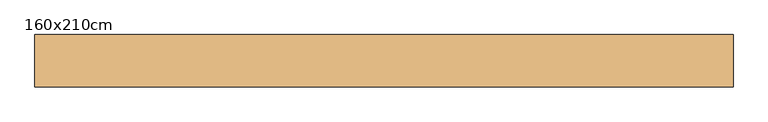
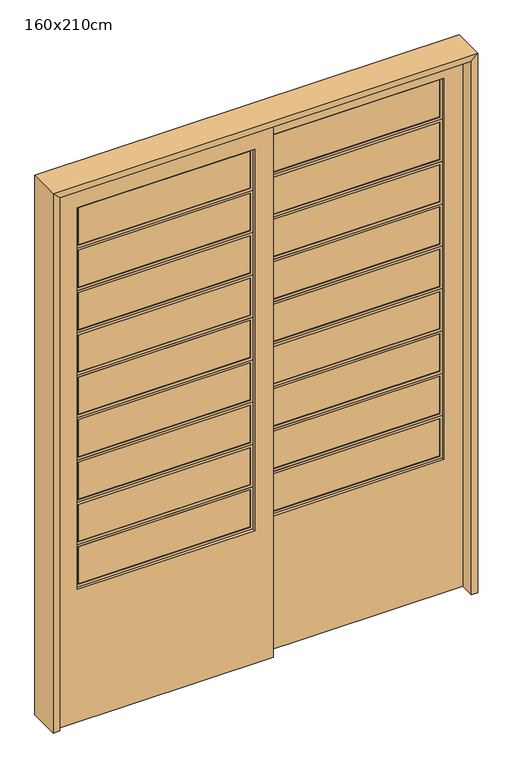
"""IFC4 building model written with IfcOpenShell, lengths in millimetres: door geometry, Porta de Correr Metálica com Divisões Horizontais : 160x210cm."""

from ifc_helpers import new_model, si_unit, frame, origin, place, context, project, spatial, polyline, outline, extrude, faceted_brep, source, transform, mapped, element, save


def door_160x210cm_b8ce621b(model_context):
    return source(origin(), model_context, "Body", "SolidModel", [
        extrude(outline(polyline([(693.0, -14.8955481), (693.0, -19.8955481), (45.0, -19.8955481), (45.0, -14.8955481), (693.0, -14.8955481)])), frame((0.0, 0.0, 1944.1111111), z_axis=(0.0, 0.0, 1.0), x_axis=(1.0, 0.0, 0.0)), (0.0, 0.0, 1.0), 149.0),
        extrude(outline(polyline([(1934.1111111, 703.0), (2103.1111111, 703.0), (2103.1111111, 35.0), (1934.1111111, 35.0), (1934.1111111, 703.0)]), holes=[polyline([(2093.1111111, 45.0), (2093.1111111, 693.0), (1944.1111111, 693.0), (1944.1111111, 45.0), (2093.1111111, 45.0)])]), frame((0.0, -22.3955481, 0.0), z_axis=(0.0, 1.0, 0.0), x_axis=(0.0, 0.0, 1.0)), (0.0, 0.0, 1.0), 10.0),
        extrude(outline(polyline([(693.0, -14.8955481), (693.0, -19.8955481), (45.0, -19.8955481), (45.0, -14.8955481), (693.0, -14.8955481)])), frame((0.0, 0.0, 1775.2222222), z_axis=(0.0, 0.0, 1.0), x_axis=(1.0, 0.0, 0.0)), (0.0, 0.0, 1.0), 149.0),
        extrude(outline(polyline([(1765.2222222, 703.0), (1934.2222222, 703.0), (1934.2222222, 35.0), (1765.2222222, 35.0), (1765.2222222, 703.0)]), holes=[polyline([(1924.2222222, 45.0), (1924.2222222, 693.0), (1775.2222222, 693.0), (1775.2222222, 45.0), (1924.2222222, 45.0)])]), frame((0.0, -22.3955481, 0.0), z_axis=(0.0, 1.0, 0.0), x_axis=(0.0, 0.0, 1.0)), (0.0, 0.0, 1.0), 10.0),
        extrude(outline(polyline([(693.0, -14.8955481), (693.0, -19.8955481), (45.0, -19.8955481), (45.0, -14.8955481), (693.0, -14.8955481)])), frame((0.0, 0.0, 1606.3333333), z_axis=(0.0, 0.0, 1.0), x_axis=(1.0, 0.0, 0.0)), (0.0, 0.0, 1.0), 149.0),
        extrude(outline(polyline([(1596.3333333, 703.0), (1765.3333333, 703.0), (1765.3333333, 35.0), (1596.3333333, 35.0), (1596.3333333, 703.0)]), holes=[polyline([(1755.3333333, 45.0), (1755.3333333, 693.0), (1606.3333333, 693.0), (1606.3333333, 45.0), (1755.3333333, 45.0)])]), frame((0.0, -22.3955481, 0.0), z_axis=(0.0, 1.0, 0.0), x_axis=(0.0, 0.0, 1.0)), (0.0, 0.0, 1.0), 10.0),
        extrude(outline(polyline([(693.0, -14.8955481), (693.0, -19.8955481), (45.0, -19.8955481), (45.0, -14.8955481), (693.0, -14.8955481)])), frame((0.0, 0.0, 1437.4444444), z_axis=(0.0, 0.0, 1.0), x_axis=(1.0, 0.0, 0.0)), (0.0, 0.0, 1.0), 149.0),
        extrude(outline(polyline([(1427.4444444, 703.0), (1596.4444444, 703.0), (1596.4444444, 35.0), (1427.4444444, 35.0), (1427.4444444, 703.0)]), holes=[polyline([(1586.4444444, 45.0), (1586.4444444, 693.0), (1437.4444444, 693.0), (1437.4444444, 45.0), (1586.4444444, 45.0)])]), frame((0.0, -22.3955481, 0.0), z_axis=(0.0, 1.0, 0.0), x_axis=(0.0, 0.0, 1.0)), (0.0, 0.0, 1.0), 10.0),
        extrude(outline(polyline([(693.0, -14.8955481), (693.0, -19.8955481), (45.0, -19.8955481), (45.0, -14.8955481), (693.0, -14.8955481)])), frame((0.0, 0.0, 1268.5555556), z_axis=(0.0, 0.0, 1.0), x_axis=(1.0, 0.0, 0.0)), (0.0, 0.0, 1.0), 149.0),
        extrude(outline(polyline([(1258.5555556, 703.0), (1427.5555556, 703.0), (1427.5555556, 35.0), (1258.5555556, 35.0), (1258.5555556, 703.0)]), holes=[polyline([(1417.5555556, 45.0), (1417.5555556, 693.0), (1268.5555556, 693.0), (1268.5555556, 45.0), (1417.5555556, 45.0)])]), frame((0.0, -22.3955481, 0.0), z_axis=(0.0, 1.0, 0.0), x_axis=(0.0, 0.0, 1.0)), (0.0, 0.0, 1.0), 10.0),
        extrude(outline(polyline([(693.0, -14.8955481), (693.0, -19.8955481), (45.0, -19.8955481), (45.0, -14.8955481), (693.0, -14.8955481)])), frame((0.0, 0.0, 1099.6666667), z_axis=(0.0, 0.0, 1.0), x_axis=(1.0, 0.0, 0.0)), (0.0, 0.0, 1.0), 149.0),
        extrude(outline(polyline([(1089.6666667, 703.0), (1258.6666667, 703.0), (1258.6666667, 35.0), (1089.6666667, 35.0), (1089.6666667, 703.0)]), holes=[polyline([(1248.6666667, 45.0), (1248.6666667, 693.0), (1099.6666667, 693.0), (1099.6666667, 45.0), (1248.6666667, 45.0)])]), frame((0.0, -22.3955481, 0.0), z_axis=(0.0, 1.0, 0.0), x_axis=(0.0, 0.0, 1.0)), (0.0, 0.0, 1.0), 10.0),
        extrude(outline(polyline([(693.0, -14.8955481), (693.0, -19.8955481), (45.0, -19.8955481), (45.0, -14.8955481), (693.0, -14.8955481)])), frame((0.0, 0.0, 930.7777778), z_axis=(0.0, 0.0, 1.0), x_axis=(1.0, 0.0, 0.0)), (0.0, 0.0, 1.0), 149.0),
        extrude(outline(polyline([(920.7777778, 703.0), (1089.7777778, 703.0), (1089.7777778, 35.0), (920.7777778, 35.0), (920.7777778, 703.0)]), holes=[polyline([(1079.7777778, 45.0), (1079.7777778, 693.0), (930.7777778, 693.0), (930.7777778, 45.0), (1079.7777778, 45.0)])]), frame((0.0, -22.3955481, 0.0), z_axis=(0.0, 1.0, 0.0), x_axis=(0.0, 0.0, 1.0)), (0.0, 0.0, 1.0), 10.0),
        extrude(outline(polyline([(693.0, -14.8955481), (693.0, -19.8955481), (45.0, -19.8955481), (45.0, -14.8955481), (693.0, -14.8955481)])), frame((0.0, 0.0, 761.8888889), z_axis=(0.0, 0.0, 1.0), x_axis=(1.0, 0.0, 0.0)), (0.0, 0.0, 1.0), 149.0),
        extrude(outline(polyline([(751.8888889, 703.0), (920.8888889, 703.0), (920.8888889, 35.0), (751.8888889, 35.0), (751.8888889, 703.0)]), holes=[polyline([(910.8888889, 45.0), (910.8888889, 693.0), (761.8888889, 693.0), (761.8888889, 45.0), (910.8888889, 45.0)])]), frame((0.0, -22.3955481, 0.0), z_axis=(0.0, 1.0, 0.0), x_axis=(0.0, 0.0, 1.0)), (0.0, 0.0, 1.0), 10.0),
        extrude(outline(polyline([(693.0, -14.8955481), (693.0, -19.8955481), (45.0, -19.8955481), (45.0, -14.8955481), (693.0, -14.8955481)])), frame((0.0, 0.0, 593.0), z_axis=(0.0, 0.0, 1.0), x_axis=(1.0, 0.0, 0.0)), (0.0, 0.0, 1.0), 149.0),
        extrude(outline(polyline([(583.0, 703.0), (752.0, 703.0), (752.0, 35.0), (583.0, 35.0), (583.0, 703.0)]), holes=[polyline([(742.0, 45.0), (742.0, 693.0), (593.0, 693.0), (593.0, 45.0), (742.0, 45.0)])]), frame((0.0, -22.3955481, 0.0), z_axis=(0.0, 1.0, 0.0), x_axis=(0.0, 0.0, 1.0)), (0.0, 0.0, 1.0), 10.0),
        extrude(outline(polyline([(-45.0, -57.1), (-45.0, -62.1), (-693.0, -62.1), (-693.0, -57.1), (-45.0, -57.1)])), frame((0.0, 0.0, 1944.1111111), z_axis=(0.0, 0.0, 1.0), x_axis=(1.0, 0.0, 0.0)), (0.0, 0.0, 1.0), 149.0),
        extrude(outline(polyline([(1934.1111111, -35.0), (2103.1111111, -35.0), (2103.1111111, -703.0), (1934.1111111, -703.0), (1934.1111111, -35.0)]), holes=[polyline([(2093.1111111, -693.0), (2093.1111111, -45.0), (1944.1111111, -45.0), (1944.1111111, -693.0), (2093.1111111, -693.0)])]), frame((0.0, -64.6, 0.0), z_axis=(0.0, 1.0, 0.0), x_axis=(0.0, 0.0, 1.0)), (0.0, 0.0, 1.0), 10.0),
        extrude(outline(polyline([(-45.0, -57.1), (-45.0, -62.1), (-693.0, -62.1), (-693.0, -57.1), (-45.0, -57.1)])), frame((0.0, 0.0, 1775.2222222), z_axis=(0.0, 0.0, 1.0), x_axis=(1.0, 0.0, 0.0)), (0.0, 0.0, 1.0), 149.0),
        extrude(outline(polyline([(1765.2222222, -35.0), (1934.2222222, -35.0), (1934.2222222, -703.0), (1765.2222222, -703.0), (1765.2222222, -35.0)]), holes=[polyline([(1924.2222222, -693.0), (1924.2222222, -45.0), (1775.2222222, -45.0), (1775.2222222, -693.0), (1924.2222222, -693.0)])]), frame((0.0, -64.6, 0.0), z_axis=(0.0, 1.0, 0.0), x_axis=(0.0, 0.0, 1.0)), (0.0, 0.0, 1.0), 10.0),
        extrude(outline(polyline([(-45.0, -57.1), (-45.0, -62.1), (-693.0, -62.1), (-693.0, -57.1), (-45.0, -57.1)])), frame((0.0, 0.0, 1606.3333333), z_axis=(0.0, 0.0, 1.0), x_axis=(1.0, 0.0, 0.0)), (0.0, 0.0, 1.0), 149.0),
        extrude(outline(polyline([(1596.3333333, -35.0), (1765.3333333, -35.0), (1765.3333333, -703.0), (1596.3333333, -703.0), (1596.3333333, -35.0)]), holes=[polyline([(1755.3333333, -693.0), (1755.3333333, -45.0), (1606.3333333, -45.0), (1606.3333333, -693.0), (1755.3333333, -693.0)])]), frame((0.0, -64.6, 0.0), z_axis=(0.0, 1.0, 0.0), x_axis=(0.0, 0.0, 1.0)), (0.0, 0.0, 1.0), 10.0),
        extrude(outline(polyline([(-45.0, -57.1), (-45.0, -62.1), (-693.0, -62.1), (-693.0, -57.1), (-45.0, -57.1)])), frame((0.0, 0.0, 1437.4444444), z_axis=(0.0, 0.0, 1.0), x_axis=(1.0, 0.0, 0.0)), (0.0, 0.0, 1.0), 149.0),
        extrude(outline(polyline([(1427.4444444, -35.0), (1596.4444444, -35.0), (1596.4444444, -703.0), (1427.4444444, -703.0), (1427.4444444, -35.0)]), holes=[polyline([(1586.4444444, -693.0), (1586.4444444, -45.0), (1437.4444444, -45.0), (1437.4444444, -693.0), (1586.4444444, -693.0)])]), frame((0.0, -64.6, 0.0), z_axis=(0.0, 1.0, 0.0), x_axis=(0.0, 0.0, 1.0)), (0.0, 0.0, 1.0), 10.0),
        extrude(outline(polyline([(-45.0, -57.1), (-45.0, -62.1), (-693.0, -62.1), (-693.0, -57.1), (-45.0, -57.1)])), frame((0.0, 0.0, 1268.5555556), z_axis=(0.0, 0.0, 1.0), x_axis=(1.0, 0.0, 0.0)), (0.0, 0.0, 1.0), 149.0),
        extrude(outline(polyline([(1258.5555556, -35.0), (1427.5555556, -35.0), (1427.5555556, -703.0), (1258.5555556, -703.0), (1258.5555556, -35.0)]), holes=[polyline([(1417.5555556, -693.0), (1417.5555556, -45.0), (1268.5555556, -45.0), (1268.5555556, -693.0), (1417.5555556, -693.0)])]), frame((0.0, -64.6, 0.0), z_axis=(0.0, 1.0, 0.0), x_axis=(0.0, 0.0, 1.0)), (0.0, 0.0, 1.0), 10.0),
        extrude(outline(polyline([(-45.0, -57.1), (-45.0, -62.1), (-693.0, -62.1), (-693.0, -57.1), (-45.0, -57.1)])), frame((0.0, 0.0, 1099.6666667), z_axis=(0.0, 0.0, 1.0), x_axis=(1.0, 0.0, 0.0)), (0.0, 0.0, 1.0), 149.0),
        extrude(outline(polyline([(1089.6666667, -35.0), (1258.6666667, -35.0), (1258.6666667, -703.0), (1089.6666667, -703.0), (1089.6666667, -35.0)]), holes=[polyline([(1248.6666667, -693.0), (1248.6666667, -45.0), (1099.6666667, -45.0), (1099.6666667, -693.0), (1248.6666667, -693.0)])]), frame((0.0, -64.6, 0.0), z_axis=(0.0, 1.0, 0.0), x_axis=(0.0, 0.0, 1.0)), (0.0, 0.0, 1.0), 10.0),
        extrude(outline(polyline([(-45.0, -57.1), (-45.0, -62.1), (-693.0, -62.1), (-693.0, -57.1), (-45.0, -57.1)])), frame((0.0, 0.0, 930.7777778), z_axis=(0.0, 0.0, 1.0), x_axis=(1.0, 0.0, 0.0)), (0.0, 0.0, 1.0), 149.0),
        extrude(outline(polyline([(920.7777778, -35.0), (1089.7777778, -35.0), (1089.7777778, -703.0), (920.7777778, -703.0), (920.7777778, -35.0)]), holes=[polyline([(1079.7777778, -693.0), (1079.7777778, -45.0), (930.7777778, -45.0), (930.7777778, -693.0), (1079.7777778, -693.0)])]), frame((0.0, -64.6, 0.0), z_axis=(0.0, 1.0, 0.0), x_axis=(0.0, 0.0, 1.0)), (0.0, 0.0, 1.0), 10.0),
        extrude(outline(polyline([(-45.0, -57.1), (-45.0, -62.1), (-693.0, -62.1), (-693.0, -57.1), (-45.0, -57.1)])), frame((0.0, 0.0, 761.8888889), z_axis=(0.0, 0.0, 1.0), x_axis=(1.0, 0.0, 0.0)), (0.0, 0.0, 1.0), 149.0),
        extrude(outline(polyline([(751.8888889, -35.0), (920.8888889, -35.0), (920.8888889, -703.0), (751.8888889, -703.0), (751.8888889, -35.0)]), holes=[polyline([(910.8888889, -693.0), (910.8888889, -45.0), (761.8888889, -45.0), (761.8888889, -693.0), (910.8888889, -693.0)])]), frame((0.0, -64.6, 0.0), z_axis=(0.0, 1.0, 0.0), x_axis=(0.0, 0.0, 1.0)), (0.0, 0.0, 1.0), 10.0),
        extrude(outline(polyline([(-45.0, -57.1), (-45.0, -62.1), (-693.0, -62.1), (-693.0, -57.1), (-45.0, -57.1)])), frame((0.0, 0.0, 593.0), z_axis=(0.0, 0.0, 1.0), x_axis=(1.0, 0.0, 0.0)), (0.0, 0.0, 1.0), 149.0),
        extrude(outline(polyline([(583.0, -35.0), (752.0, -35.0), (752.0, -703.0), (583.0, -703.0), (583.0, -35.0)]), holes=[polyline([(742.0, -693.0), (742.0, -45.0), (593.0, -45.0), (593.0, -693.0), (742.0, -693.0)])]), frame((0.0, -64.6, 0.0), z_axis=(0.0, 1.0, 0.0), x_axis=(0.0, 0.0, 1.0)), (0.0, 0.0, 1.0), 10.0),
        extrude(outline(polyline([(2173.0, -35.0), (53.0, -35.0), (53.0, 773.0), (2173.0, 773.0), (2173.0, -35.0)]), holes=[polyline([(2103.0, 35.0), (2103.0, 703.0), (583.0, 703.0), (583.0, 35.0), (2103.0, 35.0)])]), frame((0.0, -33.6, 0.0), z_axis=(0.0, 1.0, 0.0), x_axis=(0.0, 0.0, 1.0)), (0.0, 0.0, 1.0), 32.0),
        faceted_brep([(-776.0, -85.6, 50.0), (-800.0, -85.6, 50.0), (-800.0, 34.4, 50.0), (-776.0, 34.4, 50.0), (-776.0, 34.4, 2176.0), (-776.0, -85.6, 2176.0), (-800.0, 34.4, 2200.0), (-800.0, -85.6, 2200.0), (776.0, -85.6, 50.0), (776.0, 34.4, 50.0), (800.0, 34.4, 50.0), (800.0, -85.6, 50.0), (776.0, -85.6, 2176.0), (800.0, -85.6, 2200.0), (800.0, 34.4, 2200.0), (776.0, 34.4, 2176.0)], [[[0, 1, 2, 3]], [[3, 4, 5, 0]], [[2, 6, 4, 3]], [[1, 7, 6, 2]], [[0, 5, 7, 1]], [[8, 9, 10, 11]], [[12, 8, 11, 13]], [[13, 11, 10, 14]], [[14, 10, 9, 15]], [[15, 9, 8, 12]], [[4, 15, 12, 5]], [[6, 14, 15, 4]], [[7, 13, 14, 6]], [[5, 12, 13, 7]]]),
        extrude(outline(polyline([(2173.0, -773.0), (53.0, -773.0), (53.0, 35.0), (2173.0, 35.0), (2173.0, -773.0)]), holes=[polyline([(2103.0, -703.0), (2103.0, -35.0), (583.0, -35.0), (583.0, -703.0), (2103.0, -703.0)])]), frame((0.0, -75.6, 0.0), z_axis=(0.0, 1.0, 0.0), x_axis=(0.0, 0.0, 1.0)), (0.0, 0.0, 1.0), 32.6),
    ])


if __name__ == "__main__":
    model = new_model("IFC4")
    model_context = context("Model", 3, world=origin())
    ifc_project = project(units=[si_unit("LENGTHUNIT", "METRE", prefix="MILLI")], contexts=[model_context])
    site = spatial("IfcSite", under=ifc_project)
    building = spatial("IfcBuilding", under=site)
    placement = place(None, origin())
    door_160x210cm_shape = door_160x210cm_b8ce621b(model_context)
    element("IfcDoor", 1, ObjectType="Porta de Correr Metálica com Divisões Horizontais : 160x210cm", at=placement, inside=building, context=model_context, shape_type="MappedRepresentation", body=[
        mapped(door_160x210cm_shape, transform((0.0, 0.0, 0.0), x_axis=(1.0, 0.0, 0.0), y_axis=(0.0, 1.0, 0.0), z_axis=(0.0, 0.0, 1.0))),
    ])
    save(model, "model.ifc")

# Revit data of these elements
# Type "Porta de Correr Metálica com Divisões Horizontais : 160x210cm"
#   Type Mark = "PT52"
#   SINAPI = ""
#   Construction Type = "300"
#   Model = "PORTA DE CORRER"
#   Maçaneta [instance default] = ""
#   Fechadura [instance default] = ""
#   Description = "PORTA DE FERRO"
#   Vão Luz (somente para informação) = 153.20 cm
#   Tolerância Folha Vertical = 0.30 cm
#   Módulo Básico M = 10.00 cm
#   Largura de Coordenação Modular Largura CM = 160.00 cm
#   Rough Width = 160.00 cm
#   Largura Vidro = 66.80 cm
#   Altura de Coordenação Modular Largura CM = 220.00 cm
#   Rough Height = 220.00 cm
#   Altura Nominal = 211.60 cm
#   Ajuste de Coordenação Topo AC Topo = 0.00 cm
#   Ajuste de Coordenação Base AC Base = 5.00 cm
#   Ajuste de Coordenação AC = 0.00 cm
#   Tolerância Folha Horizontal = 0.30 cm
#   Largura Folha somente para informação = 80.80 cm
#   Espessura Folha = 3.20 cm
#   Maçaneta - Distância da Folha = 3.40 cm
#   Maçaneta - Altura = 100.00 cm
#   Largura Nominal (Largura Mn) = 155.20 cm
#   Distância do Nível = 0.30 cm
#   Aduela Interna Espessura = 2.40 cm
#   Aduela Externa Espessura = 3.40 cm
#   Altura Folha somente para informação = 212.00 cm
#   Height = 215.00 cm
#   Width = 160.00 cm
#   Número de Módulos Básicos nM Largura = 16
#   Número de Módulos Básicos nM Altura = 22
#   Aduela Metálica de Canto = no
#   Batente - Material [instance default] = none
#   Painel - Material [instance default] = none
#   Function = (empty or 0)
#   Wall Closure = (empty or 0)
#   Assembly Code = ""
# Element 1 (IfcDoor, "Porta de Correr Metálica com Divisões Horizontais : 160x210cm")
#   Materials on its faces: "Ferro - Pintura Esmalte", "Vidro"
# Materials
#   "Ferro - Pintura Esmalte": class "Pintura", colour RGB 255 255 255, transparency 0, Cost = 0
#   "Vidro": class "Vidro", colour RGB 230 230 230, transparency 0.75, Cost = 0
